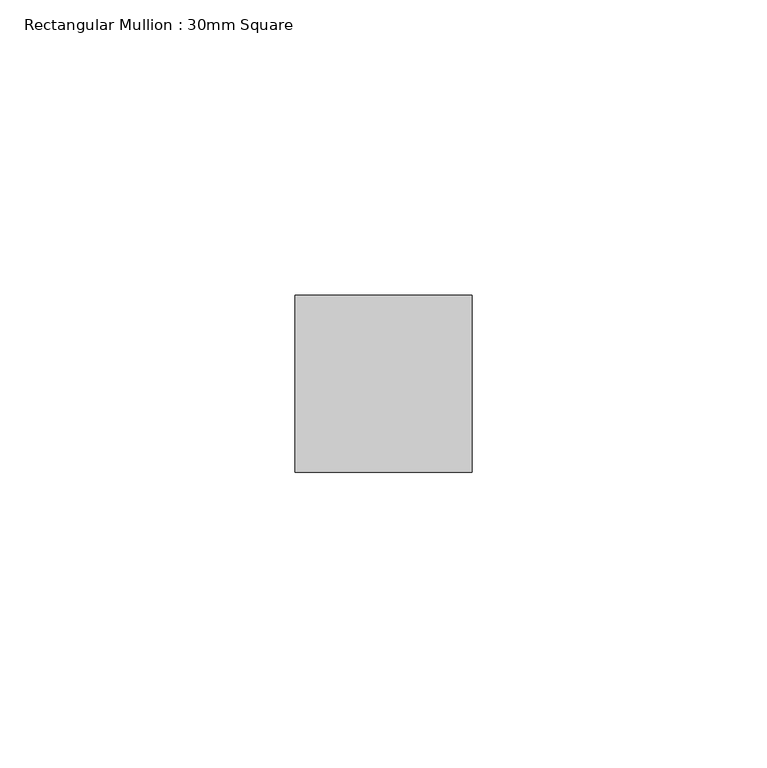
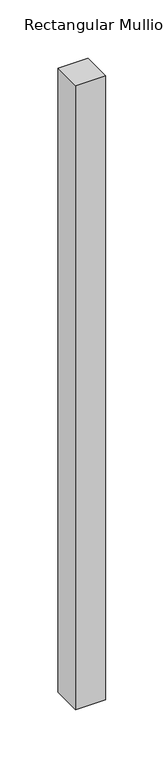
"""IFC4 building model written with IfcOpenShell, lengths in millimetres: member geometry, Rectangular Mullion : 30mm Square."""

from ifc_helpers import new_model, si_unit, frame, origin, place, context, project, spatial, polyline, outline, extrude, source, transform, mapped, element, save


def rectangular_mullion_30mm_square_92dad0e2(model_context):
    return source(origin(), model_context, "Body", "SweptSolid", [
        extrude(outline(polyline([(15.0, 15.0), (15.0, -15.0), (-15.0, -15.0), (-15.0, 15.0), (15.0, 15.0)])), frame((0.0, 0.0, -654.5999512), z_axis=(0.0, 0.0, 1.0), x_axis=(1.0, 0.0, 0.0)), (0.0, 0.0, 1.0), 654.5999512),
    ])


if __name__ == "__main__":
    model = new_model("IFC4")
    model_context = context("Model", 3, world=origin())
    ifc_project = project(units=[si_unit("LENGTHUNIT", "METRE", prefix="MILLI")], contexts=[model_context])
    site = spatial("IfcSite", under=ifc_project)
    building = spatial("IfcBuilding", under=site)
    placement = place(None, origin())
    rectangular_mullion_30mm_square_shape = rectangular_mullion_30mm_square_92dad0e2(model_context)
    element("IfcMember", 1, ObjectType="Rectangular Mullion : 30mm Square", at=placement, inside=building, context=model_context, shape_type="MappedRepresentation", body=[
        mapped(rectangular_mullion_30mm_square_shape, transform((0.0, 0.0, 0.0), x_axis=(1.0, 0.0, 0.0), y_axis=(0.0, 1.0, 0.0), z_axis=(0.0, 0.0, 1.0))),
    ])
    save(model, "model.ifc")

# Revit data of these elements
# Type "Rectangular Mullion : 30mm Square"
#   built-in parameter 1007304 = 0.0984252 (stored number, unit not read)
#   built-in parameter 1007301 = 0.0492126 (stored number, unit not read)
#   built-in parameter 1007300 = 0.0492126 (stored number, unit not read)
# Element 1 (IfcMember, "Rectangular Mullion : 30mm Square")
#   Materials on its faces: "Aluminum"
# Materials
#   "Aluminum": class "Metal", colour RGB 244 244 244, transparency 0, Description = "Aluminum 6061", Cost = 0
